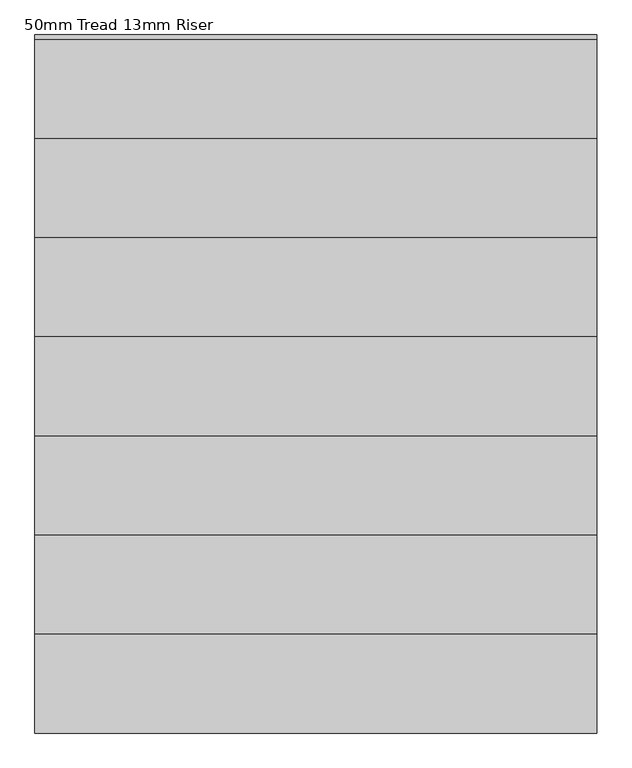
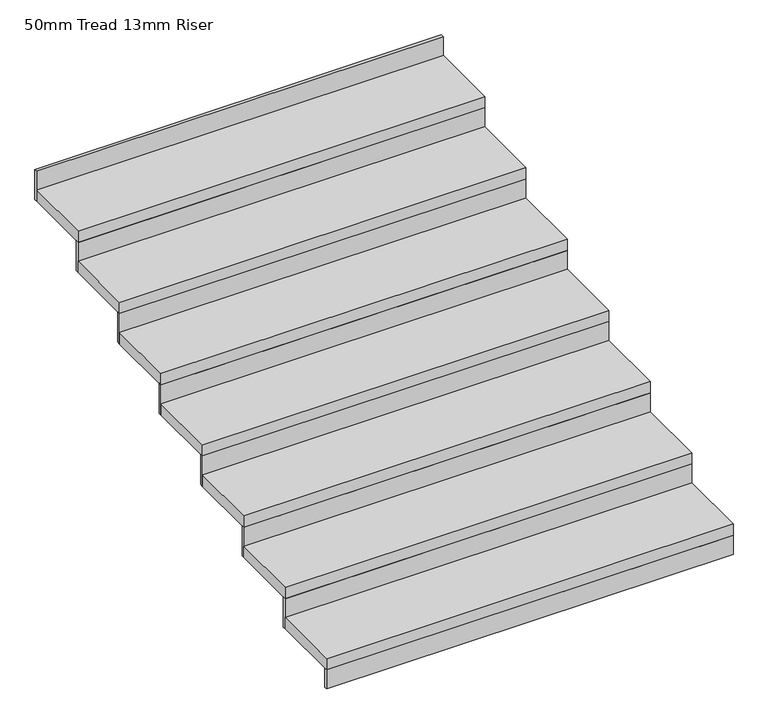
"""IFC4 building model written with IfcOpenShell, lengths in millimetres: stair flight geometry, 50mm Tread 13mm Riser."""

from ifc_helpers import new_model, si_unit, frame, origin, place, context, project, spatial, polyline, outline, extrude, source, transform, mapped, element, save


def stair_flight_50mm_tread_13mm_riser_6111fc84(model_context):
    return source(origin(), model_context, "Body", "SweptSolid", [
        extrude(outline(polyline([(-15825.2814495, -7705.5731037), (-15825.2814495, -7718.0731037), (-17525.2814495, -7718.0731037), (-17525.2814495, -7705.5731037), (-15825.2814495, -7705.5731037)])), frame((0.0, 0.0, -3200.0), z_axis=(0.0, 0.0, 1.0), x_axis=(1.0, 0.0, 0.0)), (0.0, 0.0, 1.0), 83.3333333),
        extrude(outline(polyline([(-17525.2814495, -7418.0731037), (-15825.2814495, -7418.0731037), (-15825.2814495, -7718.0731037), (-17525.2814495, -7718.0731037), (-17525.2814495, -7418.0731037)])), frame((0.0, 0.0, -3116.6666667), z_axis=(0.0, 0.0, 1.0), x_axis=(1.0, 0.0, 0.0)), (0.0, 0.0, 1.0), 50.0),
        extrude(outline(polyline([(-15825.2814495, -7405.5731037), (-15825.2814495, -7418.0731037), (-17525.2814495, -7418.0731037), (-17525.2814495, -7405.5731037), (-15825.2814495, -7405.5731037)])), frame((0.0, 0.0, -3116.6666667), z_axis=(0.0, 0.0, 1.0), x_axis=(1.0, 0.0, 0.0)), (0.0, 0.0, 1.0), 133.3333333),
        extrude(outline(polyline([(-17525.2814495, -7118.0731037), (-15825.2814495, -7118.0731037), (-15825.2814495, -7418.0731037), (-17525.2814495, -7418.0731037), (-17525.2814495, -7118.0731037)])), frame((0.0, 0.0, -2983.3333333), z_axis=(0.0, 0.0, 1.0), x_axis=(1.0, 0.0, 0.0)), (0.0, 0.0, 1.0), 50.0),
        extrude(outline(polyline([(-15825.2814495, -7105.5731037), (-15825.2814495, -7118.0731037), (-17525.2814495, -7118.0731037), (-17525.2814495, -7105.5731037), (-15825.2814495, -7105.5731037)])), frame((0.0, 0.0, -2983.3333333), z_axis=(0.0, 0.0, 1.0), x_axis=(1.0, 0.0, 0.0)), (0.0, 0.0, 1.0), 133.3333333),
        extrude(outline(polyline([(-17525.2814495, -6818.0731037), (-15825.2814495, -6818.0731037), (-15825.2814495, -7118.0731037), (-17525.2814495, -7118.0731037), (-17525.2814495, -6818.0731037)])), frame((0.0, 0.0, -2850.0), z_axis=(0.0, 0.0, 1.0), x_axis=(1.0, 0.0, 0.0)), (0.0, 0.0, 1.0), 50.0),
        extrude(outline(polyline([(-15825.2814495, -6805.5731037), (-15825.2814495, -6818.0731037), (-17525.2814495, -6818.0731037), (-17525.2814495, -6805.5731037), (-15825.2814495, -6805.5731037)])), frame((0.0, 0.0, -2850.0), z_axis=(0.0, 0.0, 1.0), x_axis=(1.0, 0.0, 0.0)), (0.0, 0.0, 1.0), 133.3333333),
        extrude(outline(polyline([(-17525.2814495, -6518.0731037), (-15825.2814495, -6518.0731037), (-15825.2814495, -6818.0731037), (-17525.2814495, -6818.0731037), (-17525.2814495, -6518.0731037)])), frame((0.0, 0.0, -2716.6666667), z_axis=(0.0, 0.0, 1.0), x_axis=(1.0, 0.0, 0.0)), (0.0, 0.0, 1.0), 50.0),
        extrude(outline(polyline([(-15825.2814495, -6505.5731037), (-15825.2814495, -6518.0731037), (-17525.2814495, -6518.0731037), (-17525.2814495, -6505.5731037), (-15825.2814495, -6505.5731037)])), frame((0.0, 0.0, -2716.6666667), z_axis=(0.0, 0.0, 1.0), x_axis=(1.0, 0.0, 0.0)), (0.0, 0.0, 1.0), 133.3333333),
        extrude(outline(polyline([(-17525.2814495, -6218.0731037), (-15825.2814495, -6218.0731037), (-15825.2814495, -6518.0731037), (-17525.2814495, -6518.0731037), (-17525.2814495, -6218.0731037)])), frame((0.0, 0.0, -2583.3333333), z_axis=(0.0, 0.0, 1.0), x_axis=(1.0, 0.0, 0.0)), (0.0, 0.0, 1.0), 50.0),
        extrude(outline(polyline([(-15825.2814495, -6205.5731037), (-15825.2814495, -6218.0731037), (-17525.2814495, -6218.0731037), (-17525.2814495, -6205.5731037), (-15825.2814495, -6205.5731037)])), frame((0.0, 0.0, -2583.3333333), z_axis=(0.0, 0.0, 1.0), x_axis=(1.0, 0.0, 0.0)), (0.0, 0.0, 1.0), 133.3333333),
        extrude(outline(polyline([(-17525.2814495, -5918.0731037), (-15825.2814495, -5918.0731037), (-15825.2814495, -6218.0731037), (-17525.2814495, -6218.0731037), (-17525.2814495, -5918.0731037)])), frame((0.0, 0.0, -2450.0), z_axis=(0.0, 0.0, 1.0), x_axis=(1.0, 0.0, 0.0)), (0.0, 0.0, 1.0), 50.0),
        extrude(outline(polyline([(-15825.2814495, -5905.5731037), (-15825.2814495, -5918.0731037), (-17525.2814495, -5918.0731037), (-17525.2814495, -5905.5731037), (-15825.2814495, -5905.5731037)])), frame((0.0, 0.0, -2450.0), z_axis=(0.0, 0.0, 1.0), x_axis=(1.0, 0.0, 0.0)), (0.0, 0.0, 1.0), 133.3333333),
        extrude(outline(polyline([(-15825.2814495, -5605.5731037), (-15825.2814495, -5618.0731037), (-17525.2814495, -5618.0731037), (-17525.2814495, -5605.5731037), (-15825.2814495, -5605.5731037)])), frame((0.0, 0.0, -2316.6666667), z_axis=(0.0, 0.0, 1.0), x_axis=(1.0, 0.0, 0.0)), (0.0, 0.0, 1.0), 133.3333333),
        extrude(outline(polyline([(-17525.2814495, -5618.0731037), (-15825.2814495, -5618.0731037), (-15825.2814495, -5918.0731037), (-17525.2814495, -5918.0731037), (-17525.2814495, -5618.0731037)])), frame((0.0, 0.0, -2316.6666667), z_axis=(0.0, 0.0, 1.0), x_axis=(1.0, 0.0, 0.0)), (0.0, 0.0, 1.0), 50.0),
    ])


if __name__ == "__main__":
    model = new_model("IFC4")
    model_context = context("Model", 3, world=origin())
    ifc_project = project(units=[si_unit("LENGTHUNIT", "METRE", prefix="MILLI")], contexts=[model_context])
    site = spatial("IfcSite", under=ifc_project)
    building = spatial("IfcBuilding", under=site)
    placement = place(None, origin())
    stair_flight_50mm_tread_13mm_riser_shape = stair_flight_50mm_tread_13mm_riser_6111fc84(model_context)
    element("IfcStairFlight", 1, ObjectType="50mm Tread 13mm Riser", at=placement, inside=building, context=model_context, shape_type="MappedRepresentation", body=[
        mapped(stair_flight_50mm_tread_13mm_riser_shape, transform((0.0, 0.0, 0.0), x_axis=(1.0, 0.0, 0.0), y_axis=(0.0, 1.0, 0.0), z_axis=(0.0, 0.0, 1.0))),
    ])
    save(model, "model.ifc")
